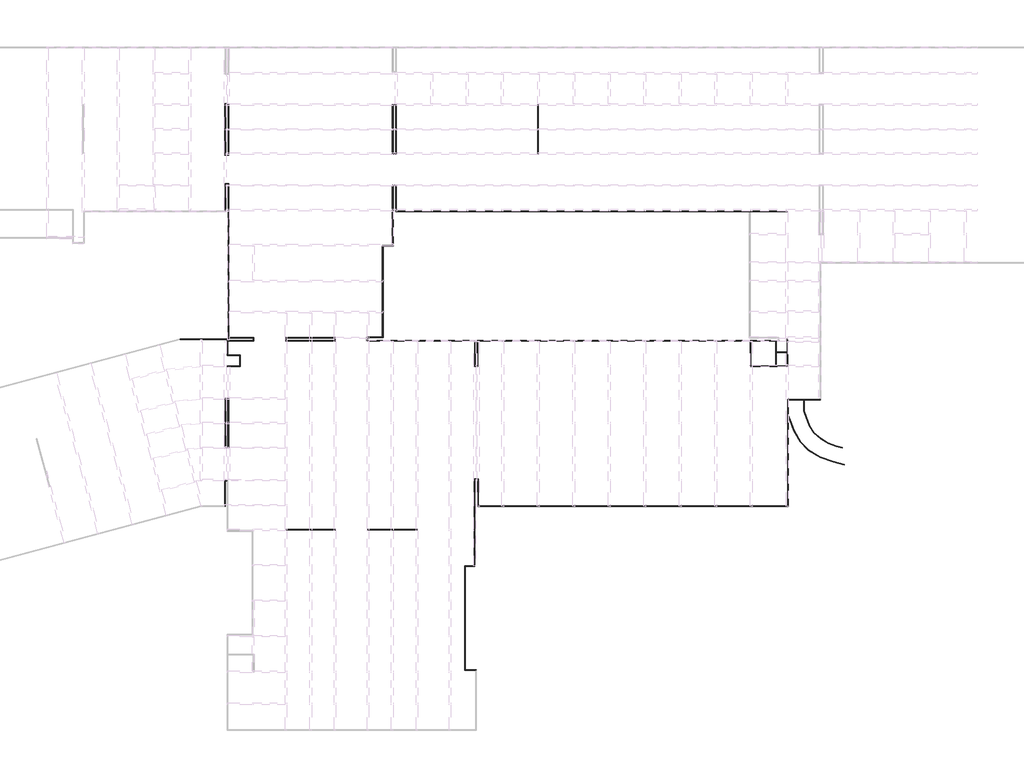
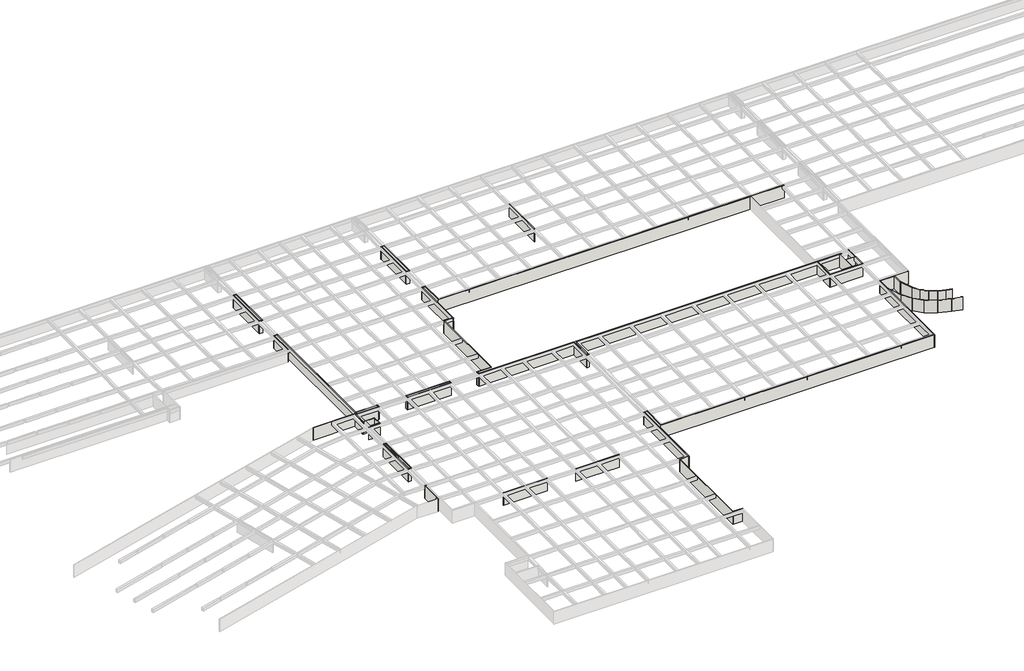
# One storey, part 2 of 14: 73 walls.
"""IFC4 building model written with IfcOpenShell, lengths in millimetres."""

import ifcopenshell
import ifcopenshell.guid

model = None  # the IFC model being written
_history = None  # IfcOwnerHistory: only IFC2X3 demands one
_inside = {}  # id of a spatial element -> (the spatial element, [elements in it])
_under = {}  # id of a project, library or spatial element -> (it, [spatial elements below it])
_declared = {}  # id of a project -> (the project, [libraries it declares])
_typed = {}  # id of a type object -> (the type object, [elements of that type])
_made_of = {}  # id of a material, layer set ... -> (it, [elements and type objects made of it])


def new_model(schema):
    """Start an empty IFC model of exactly this schema.

    Asked for "IFC4X3", IfcOpenShell would pick the latest addendum, in which some entities
    have other attributes; the version numbers below select the first issue.
    IFC2X3 requires an IfcOwnerHistory on every rooted entity: one is made here for all.
    """
    global model, _history
    if schema == "IFC4X3":
        model = ifcopenshell.file(schema_version=(4, 3, 0, 0))
    else:
        model = ifcopenshell.file(schema=schema)
    _inside.clear()
    _under.clear()
    _declared.clear()
    _typed.clear()
    _made_of.clear()
    _history = None
    if model.schema == "IFC2X3":
        org = make("IfcOrganization", Name="unknown")
        user = make(
            "IfcPersonAndOrganization",
            ThePerson=make("IfcPerson", FamilyName="unknown"),
            TheOrganization=org,
        )
        app = make(
            "IfcApplication",
            ApplicationDeveloper=org,
            Version="unknown",
            ApplicationFullName="unknown",
            ApplicationIdentifier="unknown",
        )
        _history = make(
            "IfcOwnerHistory",
            OwningUser=user,
            OwningApplication=app,
            ChangeAction="ADDED",
            CreationDate=0,
        )
    return model


def make(cls, **values):
    """One entity of the class cls with the attributes given. An attribute that is None is left unset."""
    return model.create_entity(
        cls, **{name: value for name, value in values.items() if value is not None}
    )


def rooted(cls, **values):
    """An entity with a GlobalId (a new one), such as an element, a storey or a relation."""
    return make(cls, GlobalId=ifcopenshell.guid.new(), OwnerHistory=_history, **values)


def si_unit(unit_type, name, prefix=None):
    """IfcSIUnit, for example si_unit("LENGTHUNIT", "METRE", prefix="MILLI")."""
    return make("IfcSIUnit", UnitType=unit_type, Prefix=prefix, Name=name)


def assignment(units):
    """IfcUnitAssignment: the units of a project."""
    return None if units is None else make("IfcUnitAssignment", Units=units)


def point(xyz):
    """IfcCartesianPoint."""
    return None if xyz is None else make("IfcCartesianPoint", Coordinates=xyz)


def direction(xyz):
    """IfcDirection."""
    return None if xyz is None else make("IfcDirection", DirectionRatios=xyz)


def frame(location, z_axis=None, x_axis=None):
    """IfcAxis2Placement3D, a coordinate frame: its origin and axes. An axis left out is left unset."""
    return make(
        "IfcAxis2Placement3D",
        Location=point(location),
        Axis=direction(z_axis),
        RefDirection=direction(x_axis),
    )


def origin():
    """The frame at (0, 0, 0) with its axes left unset."""
    return frame((0.0, 0.0, 0.0))


def origin_with_axes():
    """The frame at (0, 0, 0) with the z axis (0, 0, 1) and the x axis (1, 0, 0) written out."""
    return frame((0.0, 0.0, 0.0), z_axis=(0.0, 0.0, 1.0), x_axis=(1.0, 0.0, 0.0))


def place(relative_to, where):
    """IfcLocalPlacement: puts the frame where relative to a parent placement (None: the world)."""
    return make(
        "IfcLocalPlacement", PlacementRelTo=relative_to, RelativePlacement=where
    )


def context(
    kind, dimensions, precision=None, world=None, true_north=None, identifier=None
):
    """IfcGeometricRepresentationContext, for example the 3D "Model" context."""
    return make(
        "IfcGeometricRepresentationContext",
        ContextIdentifier=identifier,
        ContextType=kind,
        CoordinateSpaceDimension=dimensions,
        Precision=precision,
        WorldCoordinateSystem=world,
        TrueNorth=true_north,
    )


def project(units=None, contexts=None):
    """IfcProject with its units and contexts."""
    return rooted(
        "IfcProject",
        Name="project",
        RepresentationContexts=contexts,
        UnitsInContext=assignment(units),
    )


def spatial(cls, under=None, at=None, **own):
    """A site, building, storey or space (cls), placed at a placement, below another one or the project."""
    s = rooted(cls, ObjectPlacement=at, **own)
    if under is not None:
        _under.setdefault(under.id(), (under, []))[1].append(s)
    return s


def polyline(points):
    """IfcPolyline through the points."""
    return make("IfcPolyline", Points=[point(p) for p in points])


def outline(outer, holes=None, kind="AREA"):
    """IfcArbitraryClosedProfileDef: a profile drawn as a closed curve; with holes, ...WithVoids."""
    if holes is None:
        return make("IfcArbitraryClosedProfileDef", ProfileType=kind, OuterCurve=outer)
    return make(
        "IfcArbitraryProfileDefWithVoids",
        ProfileType=kind,
        OuterCurve=outer,
        InnerCurves=holes,
    )


def extrude(swept, where, along, depth):
    """IfcExtrudedAreaSolid: the profile swept, set in the frame where, extruded along a direction by depth."""
    return make(
        "IfcExtrudedAreaSolid",
        SweptArea=swept,
        Position=where,
        ExtrudedDirection=direction(along),
        Depth=depth,
    )


def faces_of(points, faces, orient=None, outer=None):
    """IfcFace entities. A face is a list of loops; a loop is a list of indices into points, from 0.

    orient and outer hold one flag for each loop. By default every Orientation is true, the
    first loop of a face is its IfcFaceOuterBound and the others are IfcFaceBound.
    """
    made = []
    for i, loops in enumerate(faces):
        bounds = []
        for j, loop in enumerate(loops):
            is_outer = j == 0 if outer is None else outer[i][j]
            bounds.append(
                make(
                    "IfcFaceOuterBound" if is_outer else "IfcFaceBound",
                    Bound=make("IfcPolyLoop", Polygon=[points[k] for k in loop]),
                    Orientation=True if orient is None else orient[i][j],
                )
            )
        made.append(make("IfcFace", Bounds=bounds))
    return made


def faceted_brep(points, faces, orient=None, outer=None, voids=None):
    """IfcFacetedBrep: a solid bounded by flat faces; with voids (closed shells), ...WithVoids."""
    shared = [point(p) for p in points]
    hull = make("IfcClosedShell", CfsFaces=faces_of(shared, faces, orient, outer))
    if voids is None:
        return make("IfcFacetedBrep", Outer=hull)
    return make(
        "IfcFacetedBrepWithVoids",
        Outer=hull,
        Voids=[
            make(cls, CfsFaces=faces_of(shared, fs, o, b)) for cls, fs, o, b in voids
        ],
    )


def shape(context_of_items, identifier, shape_type, items):
    """IfcShapeRepresentation: the items that make up one representation, for example the "Body"."""
    return make(
        "IfcShapeRepresentation",
        ContextOfItems=context_of_items,
        RepresentationIdentifier=identifier,
        RepresentationType=shape_type,
        Items=items,
    )


def made_of(thing, what):
    """Note that an element or type object is made of a material, layer set ...; save() writes the relation."""
    if what is not None:
        _made_of.setdefault(what.id(), (what, []))[1].append(thing)
    return thing


def element(
    cls,
    number,
    at=None,
    inside=None,
    cuts=None,
    type_object=None,
    material=None,
    context=None,
    identifier="Body",
    shape_type=None,
    held_by="IfcProductDefinitionShape",
    body=None,
    shapes=None,
    **own,
):
    """One element of the class cls, such as IfcWall. Its Tag is "e" and its number.

    at: its placement. inside: the storey or other place that contains it. cuts: it is an
    opening in that element (IfcRelVoidsElement). A single representation is given by context,
    identifier, shape_type and body (its items); several are given by shapes. held_by: the class
    of the entity that holds the representations. save() writes the other relations.
    """
    e = rooted(cls, Tag="e%d" % number, ObjectPlacement=at, **own)
    if body is not None:
        shapes = [shape(context, identifier, shape_type, body)]
    if shapes is not None:
        e.Representation = make(held_by, Representations=shapes)
    if inside is not None:
        _inside.setdefault(inside.id(), (inside, []))[1].append(e)
    if cuts is not None:
        rooted(
            "IfcRelVoidsElement", RelatingBuildingElement=cuts, RelatedOpeningElement=e
        )
    if type_object is not None:
        _typed.setdefault(type_object.id(), (type_object, []))[1].append(e)
    return made_of(e, material)


def aggregate(whole, parts):
    """IfcRelAggregates: a whole, such as a stair, and the parts it consists of."""
    return rooted("IfcRelAggregates", RelatingObject=whole, RelatedObjects=parts)


def save(model, path):
    """Write the relations noted so far, then the file.

    IfcRelAggregates (storeys below a building ...), IfcRelContainedInSpatialStructure (elements
    in a storey), IfcRelDefinesByType, IfcRelAssociatesMaterial and IfcRelDeclares: one each for
    every whole, place, type object, material and project.
    """
    for whole, parts in _under.values():
        aggregate(whole, parts)
    for where, things in _inside.values():
        rooted(
            "IfcRelContainedInSpatialStructure",
            RelatedElements=things,
            RelatingStructure=where,
        )
    for kind, things in _typed.values():
        rooted("IfcRelDefinesByType", RelatedObjects=things, RelatingType=kind)
    for what, things in _made_of.values():
        rooted("IfcRelAssociatesMaterial", RelatedObjects=things, RelatingMaterial=what)
    for by, libraries in _declared.values():
        rooted("IfcRelDeclares", RelatingContext=by, RelatedDefinitions=libraries)
    model.write(path)


model = new_model("IFC4")

# Units and contexts
model_context = context("Model", 3, world=origin())
ifc_project = project(units=[si_unit("LENGTHUNIT", "METRE", prefix="MILLI")], contexts=[model_context])

# Site, building, storey
site = spatial("IfcSite", under=ifc_project)
building = spatial("IfcBuilding", under=site)
storey = spatial("IfcBuildingStorey", under=building, Name="户型图", Elevation=0.0)

# Walls
placement = place(None, origin())
element("IfcWall", 1, ObjectType="所有墙体", at=placement, inside=storey, context=model_context, shape_type="Brep", body=[
    faceted_brep([(143467.2949044, -194796.0449275, 0.0), (136367.2949044, -194796.0449275, 0.0), (136367.2949044, -194796.0449275, 3300.0), (143467.2949044, -194796.0449275, 3300.0), (143467.2949044, -194916.0449275, 0.0), (143467.2949044, -194916.0449275, 3300.0), (140037.2949044, -194916.0449275, 3300.0), (139917.2949044, -194916.0449275, 3300.0), (136487.2949044, -194916.0449275, 3300.0), (136367.2949044, -194916.0449275, 3300.0), (136367.2949044, -194916.0449275, 0.0), (136487.2949044, -194916.0449275, 0.0), (139917.2949044, -194916.0449275, 0.0), (140037.2949044, -194916.0449275, 0.0)], [[[0, 1, 2, 3]], [[4, 5, 6, 7, 8, 9, 10, 11, 12, 13]], [[1, 0, 4, 13, 12, 11, 10]], [[3, 2, 9, 8, 7, 6, 5]], [[0, 3, 5, 4]], [[2, 1, 10, 9]]]),
])
element("IfcWall", 2, ObjectType="所有墙体", at=placement, inside=storey, context=model_context, shape_type="Brep", body=[
    faceted_brep([(136367.2949044, -194916.0449275, 0.0), (136367.2949044, -218198.950757, 0.0), (136367.2949044, -218318.950757, 0.0), (136367.2949044, -218318.950757, 3300.0), (136367.2949044, -218198.950757, 3300.0), (136367.2949044, -194916.0449275, 3300.0), (136487.2949044, -194916.0449275, 0.0), (136487.2949044, -194916.0449275, 3300.0), (136487.2949044, -198144.3728891, 3300.0), (136487.2949044, -198495.2294172, 3300.0), (136487.2949044, -218318.950757, 3300.0), (136487.2949044, -218318.950757, 0.0), (136487.2949044, -198495.2294172, 0.0), (136487.2949044, -198144.3728891, 0.0)], [[[0, 1, 2, 3, 4, 5]], [[6, 7, 8, 9, 10, 11, 12, 13]], [[2, 1, 0, 6, 13, 12, 11]], [[5, 4, 3, 10, 9, 8, 7]], [[0, 5, 7, 6]], [[3, 2, 11, 10]]]),
])
element("IfcWall", 3, ObjectType="所有墙体", at=placement, inside=storey, context=model_context, shape_type="Brep", body=[
    faceted_brep([(136367.2949044, -218198.950757, 0.0), (68337.2949044, -218198.950757, 0.0), (68217.2949044, -218198.950757, 0.0), (68217.2949044, -218198.950757, 3300.0), (68337.2949044, -218198.950757, 3300.0), (136367.2949044, -218198.950757, 3300.0), (136367.2949044, -218318.950757, 0.0), (136367.2949044, -218318.950757, 3300.0), (68217.2949044, -218318.950757, 3300.0), (68217.2949044, -218318.950757, 0.0)], [[[0, 1, 2, 3, 4, 5]], [[6, 7, 8, 9]], [[2, 1, 0, 6, 9]], [[5, 4, 3, 8, 7]], [[0, 5, 7, 6]], [[3, 2, 9, 8]]]),
])
element("IfcWall", 4, ObjectType="所有墙体", at=placement, inside=storey, context=model_context, shape_type="Brep", body=[
    faceted_brep([(68337.2949044, -218198.950757, 0.0), (68337.2949044, -212198.950757, 0.0), (68337.2949044, -212198.950757, 3300.0), (68337.2949044, -218198.950757, 3300.0), (68217.2949044, -218198.950757, 0.0), (68217.2949044, -218198.950757, 3300.0), (68217.2949044, -212318.950757, 3300.0), (68217.2949044, -212198.950757, 3300.0), (68217.2949044, -212198.950757, 0.0), (68217.2949044, -212318.950757, 0.0)], [[[0, 1, 2, 3]], [[4, 5, 6, 7, 8, 9]], [[1, 0, 4, 9, 8]], [[3, 2, 7, 6, 5]], [[0, 3, 5, 4]], [[2, 1, 8, 7]]]),
])
element("IfcWall", 5, ObjectType="所有墙体", at=placement, inside=storey, context=model_context, shape_type="Brep", body=[
    faceted_brep([(68217.2949044, -212198.950757, 0.0), (67517.2949044, -212198.950757, 0.0), (67517.2949044, -212198.950757, 3300.0), (68217.2949044, -212198.950757, 3300.0), (68217.2949044, -212318.950757, 0.0), (68217.2949044, -212318.950757, 3300.0), (67637.2949044, -212318.950757, 3300.0), (67517.2949044, -212318.950757, 3300.0), (67517.2949044, -212318.950757, 0.0), (67637.2949044, -212318.950757, 0.0)], [[[0, 1, 2, 3]], [[4, 5, 6, 7, 8, 9]], [[1, 0, 4, 9, 8]], [[3, 2, 7, 6, 5]], [[0, 3, 5, 4]], [[2, 1, 8, 7]]]),
])
element("IfcWall", 6, ObjectType="所有墙体", at=placement, inside=storey, context=model_context, shape_type="Brep", body=[
    faceted_brep([(67517.2949044, -212318.950757, 0.0), (67517.2949044, -231399.1116625, 0.0), (67517.2949044, -231519.1116625, 0.0), (67517.2949044, -231519.1116625, 3300.0), (67517.2949044, -231399.1116625, 3300.0), (67517.2949044, -212318.950757, 3300.0), (67637.2949044, -212318.950757, 0.0), (67637.2949044, -212318.950757, 3300.0), (67637.2949044, -231519.1116625, 3300.0), (67637.2949044, -231519.1116625, 0.0)], [[[0, 1, 2, 3, 4, 5]], [[6, 7, 8, 9]], [[2, 1, 0, 6, 9]], [[5, 4, 3, 8, 7]], [[0, 5, 7, 6]], [[3, 2, 9, 8]]]),
])
element("IfcWall", 7, ObjectType="所有墙体", at=placement, inside=storey, context=model_context, shape_type="Brep", body=[
    faceted_brep([(67517.2949044, -231399.1116625, 0.0), (65367.2949044, -231399.1116625, 0.0), (65367.2949044, -231399.1116625, 3300.0), (67517.2949044, -231399.1116625, 3300.0), (67517.2949044, -231519.1116625, 0.0), (67517.2949044, -231519.1116625, 3300.0), (65487.2949044, -231519.1116625, 3300.0), (65367.2949044, -231519.1116625, 3300.0), (65367.2949044, -231519.1116625, 0.0), (65487.2949044, -231519.1116625, 0.0)], [[[0, 1, 2, 3]], [[4, 5, 6, 7, 8, 9]], [[1, 0, 4, 9, 8]], [[3, 2, 7, 6, 5]], [[0, 3, 5, 4]], [[2, 1, 8, 7]]]),
])
element("IfcWall", 8, ObjectType="所有墙体", at=placement, inside=storey, context=model_context, shape_type="Brep", body=[
    faceted_brep([(65367.2949044, -231519.1116625, 0.0), (65367.2949044, -254333.1116625, 0.0), (65367.2949044, -254333.1116625, 3300.0), (65367.2949044, -231519.1116625, 3300.0), (65487.2949044, -231519.1116625, 0.0), (65487.2949044, -231519.1116625, 3300.0), (65487.2949044, -254213.1116625, 3300.0), (65487.2949044, -254333.1116625, 3300.0), (65487.2949044, -254333.1116625, 0.0), (65487.2949044, -254213.1116625, 0.0)], [[[0, 1, 2, 3]], [[4, 5, 6, 7, 8, 9]], [[1, 0, 4, 9, 8]], [[3, 2, 7, 6, 5]], [[0, 3, 5, 4]], [[2, 1, 8, 7]]]),
])
element("IfcWall", 9, ObjectType="所有墙体", at=placement, inside=storey, context=model_context, shape_type="Brep", body=[
    faceted_brep([(65487.2949044, -254333.1116625, 0.0), (67772.2743803, -254333.1116625, 0.0), (67892.2743803, -254333.1116625, 0.0), (67892.2743803, -254333.1116625, 3300.0), (67772.2743803, -254333.1116625, 3300.0), (65487.2949044, -254333.1116625, 3300.0), (65487.2949044, -254213.1116625, 0.0), (65487.2949044, -254213.1116625, 3300.0), (67892.2743803, -254213.1116625, 3300.0), (67892.2743803, -254213.1116625, 0.0)], [[[0, 1, 2, 3, 4, 5]], [[6, 7, 8, 9]], [[2, 1, 0, 6, 9]], [[5, 4, 3, 8, 7]], [[0, 5, 7, 6]], [[3, 2, 9, 8]]]),
])
element("IfcWall", 10, ObjectType="所有墙体", at=placement, inside=storey, context=model_context, shape_type="Brep", body=[
    faceted_brep([(13172.2743803, -212513.1116625, 0.0), (12672.2743803, -212513.1116625, 0.0), (12672.2743803, -212513.1116625, 3300.0), (13172.2743803, -212513.1116625, 3300.0), (13172.2743803, -212633.1116625, 0.0), (13172.2743803, -212633.1116625, 3300.0), (12792.2743803, -212633.1116625, 3300.0), (12672.2743803, -212633.1116625, 3300.0), (12672.2743803, -212633.1116625, 0.0), (12792.2743803, -212633.1116625, 0.0)], [[[0, 1, 2, 3]], [[4, 5, 6, 7, 8, 9]], [[1, 0, 4, 9, 8]], [[3, 2, 7, 6, 5]], [[0, 3, 5, 4]], [[2, 1, 8, 7]]]),
])
element("IfcWall", 11, ObjectType="所有墙体", at=placement, inside=storey, context=model_context, shape_type="Brep", body=[
    faceted_brep([(12672.2743803, -212633.1116625, 0.0), (12672.2743803, -218205.2956278, 0.0), (12672.2743803, -218325.2956278, 0.0), (12672.2743803, -218325.2956278, 3300.0), (12672.2743803, -218205.2956278, 3300.0), (12672.2743803, -212633.1116625, 3300.0), (12792.2743803, -212633.1116625, 0.0), (12792.2743803, -212633.1116625, 3300.0), (12792.2743803, -218325.2956278, 3300.0), (12792.2743803, -218325.2956278, 0.0)], [[[0, 1, 2, 3, 4, 5]], [[6, 7, 8, 9]], [[2, 1, 0, 6, 9]], [[5, 4, 3, 8, 7]], [[0, 5, 7, 6]], [[3, 2, 9, 8]]]),
])
element("IfcWall", 12, ObjectType="所有墙体", at=placement, inside=storey, context=model_context, shape_type="Brep", body=[
    faceted_brep([(2737.534582, -181627.3751505, 0.0), (13167.2949044, -181627.3751505, 0.0), (13287.2949044, -181627.3751505, 0.0), (13589.6354322, -181627.3751505, 0.0), (13589.6354322, -181627.3751505, 3300.0), (13287.2949044, -181627.3751505, 3300.0), (13167.2949044, -181627.3751505, 3300.0), (2737.534582, -181627.3751505, 3300.0), (2721.7362823, -181507.3751505, 0.0), (2721.7362823, -181507.3751505, 3300.0), (13469.6354322, -181507.3751505, 3300.0), (13589.6354322, -181507.3751505, 3300.0), (13589.6354322, -181507.3751505, 0.0), (13469.6354322, -181507.3751505, 0.0)], [[[0, 1, 2, 3, 4, 5, 6, 7]], [[8, 9, 10, 11, 12, 13]], [[3, 2, 1, 0, 8, 13, 12]], [[7, 6, 5, 4, 11, 10, 9]], [[0, 7, 9, 8]], [[4, 3, 12, 11]]]),
])
element("IfcWall", 13, ObjectType="所有墙体", at=placement, inside=storey, context=model_context, shape_type="Brep", body=[
    faceted_brep([(13589.6354322, -181507.3751505, 0.0), (13589.6354322, -181254.9655707, 0.0), (13589.6354322, -181134.9655707, 0.0), (13589.6354322, -147307.3751505, 0.0), (13589.6354322, -147307.3751505, 3300.0), (13589.6354322, -181134.9655707, 3300.0), (13589.6354322, -181254.9655707, 3300.0), (13589.6354322, -181507.3751505, 3300.0), (13469.6354322, -181507.3751505, 0.0), (13469.6354322, -181507.3751505, 3300.0), (13469.6354322, -147427.3751505, 3300.0), (13469.6354322, -147307.3751505, 3300.0), (13469.6354322, -147307.3751505, 0.0), (13469.6354322, -147427.3751505, 0.0)], [[[0, 1, 2, 3, 4, 5, 6, 7]], [[8, 9, 10, 11, 12, 13]], [[3, 2, 1, 0, 8, 13, 12]], [[7, 6, 5, 4, 11, 10, 9]], [[0, 7, 9, 8]], [[4, 3, 12, 11]]]),
])
element("IfcWall", 14, ObjectType="所有墙体", at=placement, inside=storey, context=model_context, shape_type="Brep", body=[
    faceted_brep([(13469.6354322, -147307.3751505, 0.0), (12717.2949044, -147307.3751505, 0.0), (12717.2949044, -147307.3751505, 3300.0), (13469.6354322, -147307.3751505, 3300.0), (13469.6354322, -147427.3751505, 0.0), (13469.6354322, -147427.3751505, 3300.0), (12837.2949044, -147427.3751505, 3300.0), (12717.2949044, -147427.3751505, 3300.0), (12717.2949044, -147427.3751505, 0.0), (12837.2949044, -147427.3751505, 0.0)], [[[0, 1, 2, 3]], [[4, 5, 6, 7, 8, 9]], [[1, 0, 4, 9, 8]], [[3, 2, 7, 6, 5]], [[0, 3, 5, 4]], [[2, 1, 8, 7]]]),
])
element("IfcWall", 15, ObjectType="所有墙体", at=placement, inside=storey, context=model_context, shape_type="Brep", body=[
    faceted_brep([(12717.2949044, -147427.3751505, 0.0), (12717.2949044, -153307.3751505, 0.0), (12717.2949044, -153427.3751505, 0.0), (12717.2949044, -153427.3751505, 3300.0), (12717.2949044, -153307.3751505, 3300.0), (12717.2949044, -147427.3751505, 3300.0), (12837.2949044, -147427.3751505, 0.0), (12837.2949044, -147427.3751505, 3300.0), (12837.2949044, -153427.3751505, 3300.0), (12837.2949044, -153427.3751505, 0.0)], [[[0, 1, 2, 3, 4, 5]], [[6, 7, 8, 9]], [[2, 1, 0, 6, 9]], [[5, 4, 3, 8, 7]], [[0, 5, 7, 6]], [[3, 2, 9, 8]]]),
])
element("IfcWall", 16, ObjectType="所有墙体", at=placement, inside=storey, context=model_context, shape_type="Brep", body=[
    faceted_brep([(12767.2949044, -194498.950757, 0.0), (12767.2949044, -205418.950757, 0.0), (12767.2949044, -205418.950757, 3300.0), (12767.2949044, -194498.950757, 3300.0), (12887.2949044, -194498.950757, 0.0), (12887.2949044, -194498.950757, 3300.0), (12887.2949044, -194618.950757, 3300.0), (12887.2949044, -205298.950757, 3300.0), (12887.2949044, -205418.950757, 3300.0), (12887.2949044, -205418.950757, 0.0), (12887.2949044, -205298.950757, 0.0), (12887.2949044, -194618.950757, 0.0)], [[[0, 1, 2, 3]], [[4, 5, 6, 7, 8, 9, 10, 11]], [[1, 0, 4, 11, 10, 9]], [[3, 2, 8, 7, 6, 5]], [[2, 1, 9, 8]], [[0, 3, 5, 4]]]),
])
element("IfcWall", 17, ObjectType="所有墙体", at=placement, inside=storey, context=model_context, shape_type="Brep", body=[
    faceted_brep([(12887.2949044, -205418.950757, 0.0), (13487.2949044, -205418.950757, 0.0), (13487.2949044, -205418.950757, 3300.0), (12887.2949044, -205418.950757, 3300.0), (12887.2949044, -205298.950757, 0.0), (12887.2949044, -205298.950757, 3300.0), (13367.2949044, -205298.950757, 3300.0), (13487.2949044, -205298.950757, 3300.0), (13487.2949044, -205298.950757, 0.0), (13367.2949044, -205298.950757, 0.0)], [[[0, 1, 2, 3]], [[4, 5, 6, 7, 8, 9]], [[1, 0, 4, 9, 8]], [[3, 2, 7, 6, 5]], [[0, 3, 5, 4]], [[2, 1, 8, 7]]]),
])
element("IfcWall", 18, ObjectType="所有墙体", at=placement, inside=storey, context=model_context, shape_type="Brep", body=[
    faceted_brep([(13487.2949044, -205298.950757, 0.0), (13487.2949044, -194498.950757, 0.0), (13487.2949044, -194498.950757, 3300.0), (13487.2949044, -205298.950757, 3300.0), (13367.2949044, -205298.950757, 0.0), (13367.2949044, -205298.950757, 3300.0), (13367.2949044, -194618.950757, 3300.0), (13367.2949044, -194498.950757, 3300.0), (13367.2949044, -194498.950757, 0.0), (13367.2949044, -194618.950757, 0.0)], [[[0, 1, 2, 3]], [[4, 5, 6, 7, 8, 9]], [[1, 0, 4, 9, 8]], [[3, 2, 7, 6, 5]], [[0, 3, 5, 4]], [[2, 1, 8, 7]]]),
])
element("IfcWall", 19, ObjectType="所有墙体", at=placement, inside=storey, context=model_context, shape_type="SweptSolid", body=[
    extrude(outline(polyline([(12887.2949044, -194498.950757), (13367.2949044, -194498.950757), (13367.2949044, -194618.950757), (12887.2949044, -194618.950757), (12887.2949044, -194498.950757)])), origin_with_axes(), (0.0, 0.0, 1.0), 3300.0),
])
element("IfcWall", 20, ObjectType="所有墙体", at=placement, inside=storey, context=model_context, shape_type="Brep", body=[
    faceted_brep([(13227.2949044, -187518.950757, 0.0), (16086.994268, -187518.950757, 0.0), (16086.994268, -187518.950757, 3300.0), (13227.2949044, -187518.950757, 3300.0), (13227.2949044, -187398.950757, 0.0), (13227.2949044, -187398.950757, 3300.0), (15966.994268, -187398.950757, 3300.0), (16086.994268, -187398.950757, 3300.0), (16086.994268, -187398.950757, 0.0), (15966.994268, -187398.950757, 0.0)], [[[0, 1, 2, 3]], [[4, 5, 6, 7, 8, 9]], [[1, 0, 4, 9, 8]], [[3, 2, 7, 6, 5]], [[0, 3, 5, 4]], [[2, 1, 8, 7]]]),
])
element("IfcWall", 21, ObjectType="所有墙体", at=placement, inside=storey, context=model_context, shape_type="Brep", body=[
    faceted_brep([(16086.994268, -187398.950757, 0.0), (16086.994268, -184998.950757, 0.0), (16086.994268, -184998.950757, 3300.0), (16086.994268, -187398.950757, 3300.0), (15966.994268, -187398.950757, 0.0), (15966.994268, -187398.950757, 3300.0), (15966.994268, -185118.950757, 3300.0), (15966.994268, -184998.950757, 3300.0), (15966.994268, -184998.950757, 0.0), (15966.994268, -185118.950757, 0.0)], [[[0, 1, 2, 3]], [[4, 5, 6, 7, 8, 9]], [[1, 0, 4, 9, 8]], [[3, 2, 7, 6, 5]], [[0, 3, 5, 4]], [[2, 1, 8, 7]]]),
])
element("IfcWall", 22, ObjectType="所有墙体", at=placement, inside=storey, context=model_context, shape_type="Brep", body=[
    faceted_brep([(15966.994268, -184998.950757, 0.0), (13287.2949044, -184998.950757, 0.0), (13167.2949044, -184998.950757, 0.0), (13167.2949044, -184998.950757, 3300.0), (13287.2949044, -184998.950757, 3300.0), (15966.994268, -184998.950757, 3300.0), (15966.994268, -185118.950757, 0.0), (15966.994268, -185118.950757, 3300.0), (13167.2949044, -185118.950757, 3300.0), (13167.2949044, -185118.950757, 0.0)], [[[0, 1, 2, 3, 4, 5]], [[6, 7, 8, 9]], [[2, 1, 0, 6, 9]], [[5, 4, 3, 8, 7]], [[0, 5, 7, 6]], [[3, 2, 9, 8]]]),
])
element("IfcWall", 23, ObjectType="所有墙体", at=placement, inside=storey, context=model_context, shape_type="Brep", body=[
    faceted_brep([(13287.2949044, -184998.950757, 0.0), (13287.2949044, -181918.950757, 0.0), (13287.2949044, -181798.950757, 0.0), (13287.2949044, -181627.3751505, 0.0), (13287.2949044, -181627.3751505, 3300.0), (13287.2949044, -181798.950757, 3300.0), (13287.2949044, -181918.950757, 3300.0), (13287.2949044, -184998.950757, 3300.0), (13167.2949044, -184998.950757, 0.0), (13167.2949044, -184998.950757, 3300.0), (13167.2949044, -181627.3751505, 3300.0), (13167.2949044, -181627.3751505, 0.0)], [[[0, 1, 2, 3, 4, 5, 6, 7]], [[8, 9, 10, 11]], [[3, 2, 1, 0, 8, 11]], [[7, 6, 5, 4, 10, 9]], [[0, 7, 9, 8]], [[4, 3, 11, 10]]]),
])
element("IfcWall", 24, ObjectType="所有墙体", at=placement, inside=storey, context=model_context, shape_type="Brep", body=[
    faceted_brep([(13589.6354322, -181254.9655707, 0.0), (18882.7925222, -181254.9655707, 0.0), (19002.7925222, -181254.9655707, 0.0), (19002.7925222, -181254.9655707, 3300.0), (18882.7925222, -181254.9655707, 3300.0), (13589.6354322, -181254.9655707, 3300.0), (13589.6354322, -181134.9655707, 0.0), (13589.6354322, -181134.9655707, 3300.0), (19002.7925222, -181134.9655707, 3300.0), (19002.7925222, -181134.9655707, 0.0)], [[[0, 1, 2, 3, 4, 5]], [[6, 7, 8, 9]], [[2, 1, 0, 6, 9]], [[5, 4, 3, 8, 7]], [[0, 5, 7, 6]], [[3, 2, 9, 8]]]),
])
element("IfcWall", 25, ObjectType="所有墙体", at=placement, inside=storey, context=model_context, shape_type="Brep", body=[
    faceted_brep([(18882.7925222, -181254.9655707, 0.0), (18882.7925222, -181798.950757, 0.0), (18882.7925222, -181918.950757, 0.0), (18882.7925222, -181918.950757, 3300.0), (18882.7925222, -181798.950757, 3300.0), (18882.7925222, -181254.9655707, 3300.0), (19002.7925222, -181254.9655707, 0.0), (19002.7925222, -181254.9655707, 3300.0), (19002.7925222, -181918.950757, 3300.0), (19002.7925222, -181918.950757, 0.0)], [[[0, 1, 2, 3, 4, 5]], [[6, 7, 8, 9]], [[2, 1, 0, 6, 9]], [[5, 4, 3, 8, 7]], [[0, 5, 7, 6]], [[3, 2, 9, 8]]]),
])
element("IfcWall", 26, ObjectType="所有墙体", at=placement, inside=storey, context=model_context, shape_type="SweptSolid", body=[
    extrude(outline(polyline([(13287.2949044, -181798.950757), (18882.7925222, -181798.950757), (18882.7925222, -181918.950757), (13287.2949044, -181918.950757), (13287.2949044, -181798.950757)])), origin_with_axes(), (0.0, 0.0, 1.0), 3300.0),
])
element("IfcWall", 27, ObjectType="所有墙体", at=placement, inside=storey, context=model_context, shape_type="Brep", body=[
    faceted_brep([(26067.2949044, -181184.9655707, 0.0), (26067.2949044, -181918.950757, 0.0), (26067.2949044, -181918.950757, 3300.0), (26067.2949044, -181184.9655707, 3300.0), (26187.2949044, -181184.9655707, 0.0), (26187.2949044, -181184.9655707, 3300.0), (26187.2949044, -181304.9655707, 3300.0), (26187.2949044, -181798.950757, 3300.0), (26187.2949044, -181918.950757, 3300.0), (26187.2949044, -181918.950757, 0.0), (26187.2949044, -181798.950757, 0.0), (26187.2949044, -181304.9655707, 0.0)], [[[0, 1, 2, 3]], [[4, 5, 6, 7, 8, 9, 10, 11]], [[1, 0, 4, 11, 10, 9]], [[3, 2, 8, 7, 6, 5]], [[2, 1, 9, 8]], [[0, 3, 5, 4]]]),
])
element("IfcWall", 28, ObjectType="所有墙体", at=placement, inside=storey, context=model_context, shape_type="Brep", body=[
    faceted_brep([(26187.2949044, -181918.950757, 0.0), (36992.3410651, -181918.950757, 0.0), (36992.3410651, -181918.950757, 3300.0), (26187.2949044, -181918.950757, 3300.0), (26187.2949044, -181798.950757, 0.0), (26187.2949044, -181798.950757, 3300.0), (36872.3410651, -181798.950757, 3300.0), (36992.3410651, -181798.950757, 3300.0), (36992.3410651, -181798.950757, 0.0), (36872.3410651, -181798.950757, 0.0)], [[[0, 1, 2, 3]], [[4, 5, 6, 7, 8, 9]], [[1, 0, 4, 9, 8]], [[3, 2, 7, 6, 5]], [[0, 3, 5, 4]], [[2, 1, 8, 7]]]),
])
element("IfcWall", 29, ObjectType="所有墙体", at=placement, inside=storey, context=model_context, shape_type="Brep", body=[
    faceted_brep([(36992.3410651, -181798.950757, 0.0), (36992.3410651, -181184.9655707, 0.0), (36992.3410651, -181184.9655707, 3300.0), (36992.3410651, -181798.950757, 3300.0), (36872.3410651, -181798.950757, 0.0), (36872.3410651, -181798.950757, 3300.0), (36872.3410651, -181304.9655707, 3300.0), (36872.3410651, -181184.9655707, 3300.0), (36872.3410651, -181184.9655707, 0.0), (36872.3410651, -181304.9655707, 0.0)], [[[0, 1, 2, 3]], [[4, 5, 6, 7, 8, 9]], [[1, 0, 4, 9, 8]], [[3, 2, 7, 6, 5]], [[0, 3, 5, 4]], [[2, 1, 8, 7]]]),
])
element("IfcWall", 30, ObjectType="所有墙体", at=placement, inside=storey, context=model_context, shape_type="SweptSolid", body=[
    extrude(outline(polyline([(26187.2949044, -181184.9655707), (36872.3410651, -181184.9655707), (36872.3410651, -181304.9655707), (26187.2949044, -181304.9655707), (26187.2949044, -181184.9655707)])), origin_with_axes(), (0.0, 0.0, 1.0), 3300.0),
])
element("IfcWall", 31, ObjectType="所有墙体", at=placement, inside=storey, context=model_context, shape_type="Brep", body=[
    faceted_brep([(47436.5330009, -181024.9655707, 0.0), (47316.5330009, -181024.9655707, 0.0), (43867.2949044, -181024.9655707, 0.0), (43867.2949044, -181024.9655707, 3300.0), (47316.5330009, -181024.9655707, 3300.0), (47436.5330009, -181024.9655707, 3300.0), (47436.5330009, -181144.9655707, 0.0), (47436.5330009, -181144.9655707, 3300.0), (43987.2949044, -181144.9655707, 3300.0), (43867.2949044, -181144.9655707, 3300.0), (43867.2949044, -181144.9655707, 0.0), (43987.2949044, -181144.9655707, 0.0)], [[[0, 1, 2, 3, 4, 5]], [[6, 7, 8, 9, 10, 11]], [[2, 1, 0, 6, 11, 10]], [[5, 4, 3, 9, 8, 7]], [[3, 2, 10, 9]], [[0, 5, 7, 6]]]),
])
element("IfcWall", 32, ObjectType="所有墙体", at=placement, inside=storey, context=model_context, shape_type="Brep", body=[
    faceted_brep([(43867.2949044, -181144.9655707, 0.0), (43867.2949044, -181968.950757, 0.0), (43867.2949044, -181968.950757, 3300.0), (43867.2949044, -181144.9655707, 3300.0), (43987.2949044, -181144.9655707, 0.0), (43987.2949044, -181144.9655707, 3300.0), (43987.2949044, -181848.950757, 3300.0), (43987.2949044, -181968.950757, 3300.0), (43987.2949044, -181968.950757, 0.0), (43987.2949044, -181848.950757, 0.0)], [[[0, 1, 2, 3]], [[4, 5, 6, 7, 8, 9]], [[1, 0, 4, 9, 8]], [[3, 2, 7, 6, 5]], [[0, 3, 5, 4]], [[2, 1, 8, 7]]]),
])
element("IfcWall", 33, ObjectType="所有墙体", at=placement, inside=storey, context=model_context, shape_type="Brep", body=[
    faceted_brep([(43987.2949044, -181968.950757, 0.0), (67567.2949044, -181968.950757, 0.0), (67687.2949044, -181968.950757, 0.0), (67687.2949044, -181968.950757, 3300.0), (67567.2949044, -181968.950757, 3300.0), (43987.2949044, -181968.950757, 3300.0), (43987.2949044, -181848.950757, 0.0), (43987.2949044, -181848.950757, 3300.0), (67687.2949044, -181848.950757, 3300.0), (67687.2949044, -181848.950757, 0.0)], [[[0, 1, 2, 3, 4, 5]], [[6, 7, 8, 9]], [[2, 1, 0, 6, 9]], [[5, 4, 3, 8, 7]], [[0, 5, 7, 6]], [[3, 2, 9, 8]]]),
])
element("IfcWall", 34, ObjectType="所有墙体", at=placement, inside=storey, context=model_context, shape_type="Brep", body=[
    faceted_brep([(67567.2949044, -181968.950757, 0.0), (67567.2949044, -187518.950757, 0.0), (67567.2949044, -187518.950757, 3300.0), (67567.2949044, -181968.950757, 3300.0), (67687.2949044, -181968.950757, 0.0), (67687.2949044, -181968.950757, 3300.0), (67687.2949044, -187398.950757, 3300.0), (67687.2949044, -187518.950757, 3300.0), (67687.2949044, -187518.950757, 0.0), (67687.2949044, -187398.950757, 0.0)], [[[0, 1, 2, 3]], [[4, 5, 6, 7, 8, 9]], [[1, 0, 4, 9, 8]], [[3, 2, 7, 6, 5]], [[0, 3, 5, 4]], [[2, 1, 8, 7]]]),
])
element("IfcWall", 35, ObjectType="所有墙体", at=placement, inside=storey, context=model_context, shape_type="Brep", body=[
    faceted_brep([(67687.2949044, -187518.950757, 0.0), (68228.3552546, -187518.950757, 0.0), (68228.3552546, -187518.950757, 3300.0), (67687.2949044, -187518.950757, 3300.0), (67687.2949044, -187398.950757, 0.0), (67687.2949044, -187398.950757, 3300.0), (68108.3552546, -187398.950757, 3300.0), (68228.3552546, -187398.950757, 3300.0), (68228.3552546, -187398.950757, 0.0), (68108.3552546, -187398.950757, 0.0)], [[[0, 1, 2, 3]], [[4, 5, 6, 7, 8, 9]], [[1, 0, 4, 9, 8]], [[3, 2, 7, 6, 5]], [[0, 3, 5, 4]], [[2, 1, 8, 7]]]),
])
element("IfcWall", 36, ObjectType="所有墙体", at=placement, inside=storey, context=model_context, shape_type="Brep", body=[
    faceted_brep([(68228.3552546, -187398.950757, 0.0), (68228.3552546, -181968.950757, 0.0), (68228.3552546, -181848.950757, 0.0), (68228.3552546, -181848.950757, 3300.0), (68228.3552546, -181968.950757, 3300.0), (68228.3552546, -187398.950757, 3300.0), (68108.3552546, -187398.950757, 0.0), (68108.3552546, -187398.950757, 3300.0), (68108.3552546, -181848.950757, 3300.0), (68108.3552546, -181848.950757, 0.0)], [[[0, 1, 2, 3, 4, 5]], [[6, 7, 8, 9]], [[2, 1, 0, 6, 9]], [[5, 4, 3, 8, 7]], [[0, 5, 7, 6]], [[3, 2, 9, 8]]]),
])
element("IfcWall", 37, ObjectType="所有墙体", at=placement, inside=storey, context=model_context, shape_type="Brep", body=[
    faceted_brep([(68228.3552546, -181968.950757, 0.0), (128167.631745, -181968.950757, 0.0), (128287.631745, -181968.950757, 0.0), (133768.0603935, -181968.950757, 0.0), (133888.0603935, -181968.950757, 0.0), (134428.3552546, -181968.950757, 0.0), (134428.3552546, -181968.950757, 3300.0), (133888.0603935, -181968.950757, 3300.0), (133768.0603935, -181968.950757, 3300.0), (128287.631745, -181968.950757, 3300.0), (128167.631745, -181968.950757, 3300.0), (68228.3552546, -181968.950757, 3300.0), (68228.3552546, -181848.950757, 0.0), (68228.3552546, -181848.950757, 3300.0), (134308.3552546, -181848.950757, 3300.0), (134428.3552546, -181848.950757, 3300.0), (134428.3552546, -181848.950757, 0.0), (134308.3552546, -181848.950757, 0.0)], [[[0, 1, 2, 3, 4, 5, 6, 7, 8, 9, 10, 11]], [[12, 13, 14, 15, 16, 17]], [[5, 4, 3, 2, 1, 0, 12, 17, 16]], [[11, 10, 9, 8, 7, 6, 15, 14, 13]], [[0, 11, 13, 12]], [[6, 5, 16, 15]]]),
])
element("IfcWall", 38, ObjectType="所有墙体", at=placement, inside=storey, context=model_context, shape_type="Brep", body=[
    faceted_brep([(50267.2949044, -153418.950757, 0.0), (127967.2949044, -153418.950757, 0.0), (128087.2949044, -153418.950757, 0.0), (136427.2949044, -153418.950757, 0.0), (136427.2949044, -153418.950757, 3300.0), (128087.2949044, -153418.950757, 3300.0), (127967.2949044, -153418.950757, 3300.0), (50267.2949044, -153418.950757, 3300.0), (50267.2949044, -153298.950757, 0.0), (50267.2949044, -153298.950757, 3300.0), (50387.2949044, -153298.950757, 3300.0), (136427.2949044, -153298.950757, 3300.0), (136427.2949044, -153298.950757, 0.0), (50387.2949044, -153298.950757, 0.0)], [[[0, 1, 2, 3, 4, 5, 6, 7]], [[8, 9, 10, 11, 12, 13]], [[3, 2, 1, 0, 8, 13, 12]], [[4, 3, 12, 11]], [[7, 6, 5, 4, 11, 10, 9]], [[0, 7, 9, 8]]]),
])
element("IfcWall", 39, ObjectType="所有墙体", at=placement, inside=storey, context=model_context, shape_type="Brep", body=[
    faceted_brep([(50387.2949044, -153298.950757, 0.0), (50387.2949044, -147598.950757, 0.0), (50387.2949044, -147598.950757, 3300.0), (50387.2949044, -153298.950757, 3300.0), (50267.2949044, -153298.950757, 0.0), (50267.2949044, -153298.950757, 3300.0), (50267.2949044, -147718.950757, 3300.0), (50267.2949044, -147598.950757, 3300.0), (50267.2949044, -147598.950757, 0.0), (50267.2949044, -147718.950757, 0.0)], [[[0, 1, 2, 3]], [[4, 5, 6, 7, 8, 9]], [[1, 0, 4, 9, 8]], [[3, 2, 7, 6, 5]], [[0, 3, 5, 4]], [[2, 1, 8, 7]]]),
])
element("IfcWall", 40, ObjectType="所有墙体", at=placement, inside=storey, context=model_context, shape_type="Brep", body=[
    faceted_brep([(50267.2949044, -147598.950757, 0.0), (49516.5330009, -147598.950757, 0.0), (49516.5330009, -147598.950757, 3300.0), (50267.2949044, -147598.950757, 3300.0), (50267.2949044, -147718.950757, 0.0), (50267.2949044, -147718.950757, 3300.0), (49636.5330009, -147718.950757, 3300.0), (49516.5330009, -147718.950757, 3300.0), (49516.5330009, -147718.950757, 0.0), (49636.5330009, -147718.950757, 0.0)], [[[0, 1, 2, 3]], [[4, 5, 6, 7, 8, 9]], [[1, 0, 4, 9, 8]], [[3, 2, 7, 6, 5]], [[0, 3, 5, 4]], [[2, 1, 8, 7]]]),
])
element("IfcWall", 41, ObjectType="所有墙体", at=placement, inside=storey, context=model_context, shape_type="Brep", body=[
    faceted_brep([(49516.5330009, -147718.950757, 0.0), (49516.5330009, -160898.950757, 0.0), (49516.5330009, -161018.950757, 0.0), (49516.5330009, -161018.950757, 3300.0), (49516.5330009, -160898.950757, 3300.0), (49516.5330009, -147718.950757, 3300.0), (49636.5330009, -147718.950757, 0.0), (49636.5330009, -147718.950757, 3300.0), (49636.5330009, -161018.950757, 3300.0), (49636.5330009, -161018.950757, 0.0)], [[[0, 1, 2, 3, 4, 5]], [[6, 7, 8, 9]], [[2, 1, 0, 6, 9]], [[5, 4, 3, 8, 7]], [[0, 5, 7, 6]], [[3, 2, 9, 8]]]),
])
element("IfcWall", 42, ObjectType="所有墙体", at=placement, inside=storey, context=model_context, shape_type="Brep", body=[
    faceted_brep([(49516.5330009, -160898.950757, 0.0), (47316.5330009, -160898.950757, 0.0), (47316.5330009, -160898.950757, 3300.0), (49516.5330009, -160898.950757, 3300.0), (49516.5330009, -161018.950757, 0.0), (49516.5330009, -161018.950757, 3300.0), (47436.5330009, -161018.950757, 3300.0), (47316.5330009, -161018.950757, 3300.0), (47316.5330009, -161018.950757, 0.0), (47436.5330009, -161018.950757, 0.0)], [[[0, 1, 2, 3]], [[4, 5, 6, 7, 8, 9]], [[1, 0, 4, 9, 8]], [[3, 2, 7, 6, 5]], [[0, 3, 5, 4]], [[2, 1, 8, 7]]]),
])
element("IfcWall", 43, ObjectType="所有墙体", at=placement, inside=storey, context=model_context, shape_type="SweptSolid", body=[
    extrude(outline(polyline([(47316.5330009, -181024.9655707), (47316.5330009, -161018.950757), (47436.5330009, -161018.950757), (47436.5330009, -181024.9655707), (47316.5330009, -181024.9655707)])), origin_with_axes(), (0.0, 0.0, 1.0), 3300.0),
])
element("IfcWall", 44, ObjectType="所有墙体", at=placement, inside=storey, context=model_context, shape_type="Brep", body=[
    faceted_brep([(12711.7961793, -141080.0179086, 0.0), (13537.2949044, -141080.0179086, 0.0), (13537.2949044, -141080.0179086, 3300.0), (12711.7961793, -141080.0179086, 3300.0), (12711.7961793, -140960.0179086, 0.0), (12711.7961793, -140960.0179086, 3300.0), (12831.7961793, -140960.0179086, 3300.0), (13417.2949044, -140960.0179086, 3300.0), (13537.2949044, -140960.0179086, 3300.0), (13537.2949044, -140960.0179086, 0.0), (13417.2949044, -140960.0179086, 0.0), (12831.7961793, -140960.0179086, 0.0)], [[[0, 1, 2, 3]], [[4, 5, 6, 7, 8, 9, 10, 11]], [[1, 0, 4, 11, 10, 9]], [[3, 2, 8, 7, 6, 5]], [[2, 1, 9, 8]], [[0, 3, 5, 4]]]),
])
element("IfcWall", 45, ObjectType="所有墙体", at=placement, inside=storey, context=model_context, shape_type="Brep", body=[
    faceted_brep([(13537.2949044, -140960.0179086, 0.0), (13537.2949044, -129760.0179086, 0.0), (13537.2949044, -129760.0179086, 3300.0), (13537.2949044, -140960.0179086, 3300.0), (13417.2949044, -140960.0179086, 0.0), (13417.2949044, -140960.0179086, 3300.0), (13417.2949044, -129880.0179086, 3300.0), (13417.2949044, -129760.0179086, 3300.0), (13417.2949044, -129760.0179086, 0.0), (13417.2949044, -129880.0179086, 0.0)], [[[0, 1, 2, 3]], [[4, 5, 6, 7, 8, 9]], [[1, 0, 4, 9, 8]], [[3, 2, 7, 6, 5]], [[0, 3, 5, 4]], [[2, 1, 8, 7]]]),
])
element("IfcWall", 46, ObjectType="所有墙体", at=placement, inside=storey, context=model_context, shape_type="Brep", body=[
    faceted_brep([(13417.2949044, -129760.0179086, 0.0), (12711.7961793, -129760.0179086, 0.0), (12711.7961793, -129760.0179086, 3300.0), (13417.2949044, -129760.0179086, 3300.0), (13417.2949044, -129880.0179086, 0.0), (13417.2949044, -129880.0179086, 3300.0), (12831.7961793, -129880.0179086, 3300.0), (12711.7961793, -129880.0179086, 3300.0), (12711.7961793, -129880.0179086, 0.0), (12831.7961793, -129880.0179086, 0.0)], [[[0, 1, 2, 3]], [[4, 5, 6, 7, 8, 9]], [[1, 0, 4, 9, 8]], [[3, 2, 7, 6, 5]], [[0, 3, 5, 4]], [[2, 1, 8, 7]]]),
])
element("IfcWall", 47, ObjectType="所有墙体", at=placement, inside=storey, context=model_context, shape_type="SweptSolid", body=[
    extrude(outline(polyline([(12711.7961793, -140960.0179086), (12711.7961793, -129880.0179086), (12831.7961793, -129880.0179086), (12831.7961793, -140960.0179086), (12711.7961793, -140960.0179086)])), origin_with_axes(), (0.0, 0.0, 1.0), 3300.0),
])
element("IfcWall", 48, ObjectType="所有墙体", at=placement, inside=storey, context=model_context, shape_type="Brep", body=[
    faceted_brep([(49516.5330009, -140818.950757, 0.0), (50337.2949044, -140818.950757, 0.0), (50337.2949044, -140818.950757, 3300.0), (49516.5330009, -140818.950757, 3300.0), (49516.5330009, -140698.950757, 0.0), (49516.5330009, -140698.950757, 3300.0), (49636.5330009, -140698.950757, 3300.0), (50217.2949044, -140698.950757, 3300.0), (50337.2949044, -140698.950757, 3300.0), (50337.2949044, -140698.950757, 0.0), (50217.2949044, -140698.950757, 0.0), (49636.5330009, -140698.950757, 0.0)], [[[0, 1, 2, 3]], [[4, 5, 6, 7, 8, 9, 10, 11]], [[1, 0, 4, 11, 10, 9]], [[3, 2, 8, 7, 6, 5]], [[2, 1, 9, 8]], [[0, 3, 5, 4]]]),
])
element("IfcWall", 49, ObjectType="所有墙体", at=placement, inside=storey, context=model_context, shape_type="Brep", body=[
    faceted_brep([(50337.2949044, -140698.950757, 0.0), (50337.2949044, -129898.950757, 0.0), (50337.2949044, -129898.950757, 3300.0), (50337.2949044, -140698.950757, 3300.0), (50217.2949044, -140698.950757, 0.0), (50217.2949044, -140698.950757, 3300.0), (50217.2949044, -130018.950757, 3300.0), (50217.2949044, -129898.950757, 3300.0), (50217.2949044, -129898.950757, 0.0), (50217.2949044, -130018.950757, 0.0)], [[[0, 1, 2, 3]], [[4, 5, 6, 7, 8, 9]], [[1, 0, 4, 9, 8]], [[3, 2, 7, 6, 5]], [[0, 3, 5, 4]], [[2, 1, 8, 7]]]),
])
element("IfcWall", 50, ObjectType="所有墙体", at=placement, inside=storey, context=model_context, shape_type="Brep", body=[
    faceted_brep([(50217.2949044, -129898.950757, 0.0), (49516.5330009, -129898.950757, 0.0), (49516.5330009, -129898.950757, 3300.0), (50217.2949044, -129898.950757, 3300.0), (50217.2949044, -130018.950757, 0.0), (50217.2949044, -130018.950757, 3300.0), (49636.5330009, -130018.950757, 3300.0), (49516.5330009, -130018.950757, 3300.0), (49516.5330009, -130018.950757, 0.0), (49636.5330009, -130018.950757, 0.0)], [[[0, 1, 2, 3]], [[4, 5, 6, 7, 8, 9]], [[1, 0, 4, 9, 8]], [[3, 2, 7, 6, 5]], [[0, 3, 5, 4]], [[2, 1, 8, 7]]]),
])
element("IfcWall", 51, ObjectType="所有墙体", at=placement, inside=storey, context=model_context, shape_type="SweptSolid", body=[
    extrude(outline(polyline([(49516.5330009, -140698.950757), (49516.5330009, -130018.950757), (49636.5330009, -130018.950757), (49636.5330009, -140698.950757), (49516.5330009, -140698.950757)])), origin_with_axes(), (0.0, 0.0, 1.0), 3300.0),
])
element("IfcWall", 52, ObjectType="所有墙体", at=placement, inside=storey, context=model_context, shape_type="SweptSolid", body=[
    extrude(outline(polyline([(81467.4871398, -140758.950757), (81467.4871398, -129958.950757), (81587.4871398, -129958.950757), (81587.4871398, -140758.950757), (81467.4871398, -140758.950757)])), origin_with_axes(), (0.0, 0.0, 1.0), 3300.0),
])
element("IfcWall", 53, ObjectType="所有墙体", at=placement, inside=storey, context=model_context, shape_type="SweptSolid", body=[
    extrude(outline(polyline([(37027.2949044, -223421.814057), (26127.2949044, -223421.814057), (26127.2949044, -223301.814057), (37027.2949044, -223301.814057), (37027.2949044, -223421.814057)])), origin_with_axes(), (0.0, 0.0, 1.0), 3300.0),
])
element("IfcWall", 54, ObjectType="所有墙体", at=placement, inside=storey, context=model_context, shape_type="SweptSolid", body=[
    extrude(outline(polyline([(54927.2949044, -223421.814057), (44127.2949044, -223421.814057), (44127.2949044, -223301.814057), (54927.2949044, -223301.814057), (54927.2949044, -223421.814057)])), origin_with_axes(), (0.0, 0.0, 1.0), 3300.0),
])
element("IfcWall", 55, ObjectType="所有墙体", at=placement, inside=storey, context=model_context, shape_type="Brep", body=[
    faceted_brep([(128167.631745, -181968.950757, 0.0), (128167.631745, -187518.950757, 0.0), (128167.631745, -187518.950757, 3300.0), (128167.631745, -181968.950757, 3300.0), (128287.631745, -181968.950757, 0.0), (128287.631745, -181968.950757, 3300.0), (128287.631745, -187398.950757, 3300.0), (128287.631745, -187518.950757, 3300.0), (128287.631745, -187518.950757, 0.0), (128287.631745, -187398.950757, 0.0)], [[[0, 1, 2, 3]], [[4, 5, 6, 7, 8, 9]], [[1, 0, 4, 9, 8]], [[3, 2, 7, 6, 5]], [[0, 3, 5, 4]], [[2, 1, 8, 7]]]),
])
element("IfcWall", 56, ObjectType="所有墙体", at=placement, inside=storey, context=model_context, shape_type="Brep", body=[
    faceted_brep([(128287.631745, -187518.950757, 0.0), (136407.2949044, -187518.950757, 0.0), (136407.2949044, -187518.950757, 3300.0), (128287.631745, -187518.950757, 3300.0), (128287.631745, -187398.950757, 0.0), (128287.631745, -187398.950757, 3300.0), (133768.0603935, -187398.950757, 3300.0), (133888.0603935, -187398.950757, 3300.0), (136287.2949044, -187398.950757, 3300.0), (136407.2949044, -187398.950757, 3300.0), (136407.2949044, -187398.950757, 0.0), (136287.2949044, -187398.950757, 0.0), (133888.0603935, -187398.950757, 0.0), (133768.0603935, -187398.950757, 0.0)], [[[0, 1, 2, 3]], [[4, 5, 6, 7, 8, 9, 10, 11, 12, 13]], [[1, 0, 4, 13, 12, 11, 10]], [[3, 2, 9, 8, 7, 6, 5]], [[0, 3, 5, 4]], [[2, 1, 10, 9]]]),
])
element("IfcWall", 57, ObjectType="所有墙体", at=placement, inside=storey, context=model_context, shape_type="Brep", body=[
    faceted_brep([(136407.2949044, -187398.950757, 0.0), (136407.2949044, -181358.950757, 0.0), (136407.2949044, -181358.950757, 3300.0), (136407.2949044, -187398.950757, 3300.0), (136287.2949044, -187398.950757, 0.0), (136287.2949044, -187398.950757, 3300.0), (136287.2949044, -184418.950757, 3300.0), (136287.2949044, -184298.950757, 3300.0), (136287.2949044, -181358.950757, 3300.0), (136287.2949044, -181358.950757, 0.0), (136287.2949044, -184298.950757, 0.0), (136287.2949044, -184418.950757, 0.0)], [[[0, 1, 2, 3]], [[4, 5, 6, 7, 8, 9, 10, 11]], [[1, 0, 4, 11, 10, 9]], [[2, 1, 9, 8]], [[3, 2, 8, 7, 6, 5]], [[0, 3, 5, 4]]]),
])
element("IfcWall", 58, ObjectType="所有墙体", at=placement, inside=storey, context=model_context, shape_type="Brep", body=[
    faceted_brep([(133768.0603935, -181968.950757, 0.0), (133768.0603935, -187398.950757, 0.0), (133768.0603935, -187398.950757, 3300.0), (133768.0603935, -181968.950757, 3300.0), (133888.0603935, -181968.950757, 0.0), (133888.0603935, -181968.950757, 3300.0), (133888.0603935, -184298.950757, 3300.0), (133888.0603935, -184418.950757, 3300.0), (133888.0603935, -187398.950757, 3300.0), (133888.0603935, -187398.950757, 0.0), (133888.0603935, -184418.950757, 0.0), (133888.0603935, -184298.950757, 0.0)], [[[0, 1, 2, 3]], [[4, 5, 6, 7, 8, 9, 10, 11]], [[1, 0, 4, 11, 10, 9]], [[3, 2, 8, 7, 6, 5]], [[2, 1, 9, 8]], [[0, 3, 5, 4]]]),
])
element("IfcWall", 59, ObjectType="所有墙体", at=placement, inside=storey, context=model_context, shape_type="SweptSolid", body=[
    extrude(outline(polyline([(136287.2949044, -184418.950757), (133888.0603935, -184418.950757), (133888.0603935, -184298.950757), (136287.2949044, -184298.950757), (136287.2949044, -184418.950757)])), origin_with_axes(), (0.0, 0.0, 1.0), 3300.0),
])
element("IfcWall", 60, ObjectType="所有墙体", at=placement, inside=storey, context=model_context, shape_type="SweptSolid", body=[
    extrude(outline(polyline([(136781.3622365, -199303.1727717), (136487.2949044, -198495.2294172), (136487.2949044, -198144.3728891), (136894.0759164, -199261.9945342), (136781.3622365, -199303.1727717)])), origin_with_axes(), (0.0, 0.0, 1.0), 3300.0),
])
element("IfcWall", 61, ObjectType="所有墙体", at=placement, inside=storey, context=model_context, shape_type="SweptSolid", body=[
    extrude(outline(polyline([(137645.8016972, -201660.5160969), (136781.3622365, -199303.1727717), (136894.0759164, -199261.9945342), (137754.5834402, -201608.6153905), (137645.8016972, -201660.5160969)])), origin_with_axes(), (0.0, 0.0, 1.0), 3300.0),
])
element("IfcWall", 62, ObjectType="所有墙体", at=placement, inside=storey, context=model_context, shape_type="SweptSolid", body=[
    extrude(outline(polyline([(139140.6673119, -204160.789019), (137645.8016972, -201660.5160969), (137754.5834402, -201608.6153905), (139236.0331602, -204086.4492399), (139140.6673119, -204160.789019)])), origin_with_axes(), (0.0, 0.0, 1.0), 3300.0),
])
element("IfcWall", 63, ObjectType="所有墙体", at=placement, inside=storey, context=model_context, shape_type="SweptSolid", body=[
    extrude(outline(polyline([(140918.5295066, -205938.6512137), (139140.6673119, -204160.789019), (139236.0331602, -204086.4492399), (140993.7048715, -205844.1209511), (140918.5295066, -205938.6512137)])), origin_with_axes(), (0.0, 0.0, 1.0), 3300.0),
])
element("IfcWall", 64, ObjectType="所有墙体", at=placement, inside=storey, context=model_context, shape_type="SweptSolid", body=[
    extrude(outline(polyline([(143474.9856085, -207535.3007897), (140918.5295066, -205938.6512137), (140993.7048715, -205844.1209511), (143527.2702617, -207426.4739995), (143474.9856085, -207535.3007897)])), origin_with_axes(), (0.0, 0.0, 1.0), 3300.0),
])
element("IfcWall", 65, ObjectType="所有墙体", at=placement, inside=storey, context=model_context, shape_type="SweptSolid", body=[
    extrude(outline(polyline([(146378.3647027, -208554.0882683), (143474.9856085, -207535.3007897), (143527.2702617, -207426.4739995), (146411.9685128, -208438.7064233), (146378.3647027, -208554.0882683)])), origin_with_axes(), (0.0, 0.0, 1.0), 3300.0),
])
element("IfcWall", 66, ObjectType="所有墙体", at=placement, inside=storey, context=model_context, shape_type="SweptSolid", body=[
    extrude(outline(polyline([(148809.0616975, -209121.4968069), (146378.3647027, -208554.0882683), (146411.9685128, -208438.7064233), (148836.340463, -209004.6384784), (148809.0616975, -209121.4968069)])), origin_with_axes(), (0.0, 0.0, 1.0), 3300.0),
])
element("IfcWall", 67, ObjectType="所有墙体", at=placement, inside=storey, context=model_context, shape_type="Brep", body=[
    faceted_brep([(139917.2949044, -194916.0449275, 0.0), (139917.2949044, -197266.6245463, 0.0), (139917.2949044, -197266.6245463, 3300.0), (139917.2949044, -194916.0449275, 3300.0), (140037.2949044, -194916.0449275, 0.0), (140037.2949044, -194916.0449275, 3300.0), (140037.2949044, -197245.4653086, 3300.0), (140037.2949044, -197596.3218367, 3300.0), (140037.2949044, -197596.3218367, 0.0), (140037.2949044, -197245.4653086, 0.0)], [[[0, 1, 2, 3]], [[4, 5, 6, 7, 8, 9]], [[1, 0, 4, 9, 8]], [[3, 2, 7, 6, 5]], [[0, 3, 5, 4]], [[2, 1, 8, 7]]]),
])
element("IfcWall", 68, ObjectType="所有墙体", at=placement, inside=storey, context=model_context, shape_type="SweptSolid", body=[
    extrude(outline(polyline([(141135.1435175, -200612.6361109), (140037.2949044, -197596.3218367), (140037.2949044, -197245.4653086), (141244.0000941, -200560.8605693), (141135.1435175, -200612.6361109)])), origin_with_axes(), (0.0, 0.0, 1.0), 3300.0),
])
element("IfcWall", 69, ObjectType="所有墙体", at=placement, inside=storey, context=model_context, shape_type="SweptSolid", body=[
    extrude(outline(polyline([(142066.9453077, -202171.1432851), (141135.1435175, -200612.6361109), (141244.0000941, -200560.8605693), (142159.5664427, -202092.2127706), (142066.9453077, -202171.1432851)])), origin_with_axes(), (0.0, 0.0, 1.0), 3300.0),
])
element("IfcWall", 70, ObjectType="所有墙体", at=placement, inside=storey, context=model_context, shape_type="SweptSolid", body=[
    extrude(outline(polyline([(143609.9967355, -203465.917169), (142066.9453077, -202171.1432851), (142159.5664427, -202092.2127706), (143680.6927874, -203368.5893254), (143609.9967355, -203465.917169)])), origin_with_axes(), (0.0, 0.0, 1.0), 3300.0),
])
element("IfcWall", 71, ObjectType="所有墙体", at=placement, inside=storey, context=model_context, shape_type="SweptSolid", body=[
    extrude(outline(polyline([(145230.720829, -204478.1498589), (143609.9967355, -203465.917169), (143680.6927874, -203368.5893254), (145283.0054821, -204369.3230688), (145230.720829, -204478.1498589)])), origin_with_axes(), (0.0, 0.0, 1.0), 3300.0),
])
element("IfcWall", 72, ObjectType="所有墙体", at=placement, inside=storey, context=model_context, shape_type="SweptSolid", body=[
    extrude(outline(polyline([(147030.480479, -205109.6804088), (145230.720829, -204478.1498589), (145283.0054821, -204369.3230688), (147064.0842891, -204994.2985639), (147030.480479, -205109.6804088)])), origin_with_axes(), (0.0, 0.0, 1.0), 3300.0),
])
element("IfcWall", 73, ObjectType="所有墙体", at=placement, inside=storey, context=model_context, shape_type="SweptSolid", body=[
    extrude(outline(polyline([(148331.4813088, -205413.3788876), (147030.480479, -205109.6804088), (147064.0842891, -204994.2985639), (148358.7600744, -205296.520559), (148331.4813088, -205413.3788876)])), origin_with_axes(), (0.0, 0.0, 1.0), 3300.0),
])

save(model, "model.ifc")

# Revit data of these elements
# Type "所有墙体"
#   Layers, outside or top first: 120 mm "默认" (function 1)
# Elements 1, 2, 3, 4, 5, 6, 7, 8, 9, 10, 11, 12, 13, 14, 15, 16, 17, 18, 19, 20, 21, 22, 23, 24, 25, 26, 27, 28, 29, 30, 31, 32, 33, 34, 35, 36, 37, 38, 39, 40, 41, 42, 43, 44, 45, 46, 47, 48, 49, 50, 51, 52, 53, 54, 55, 56, 57, 58, 59, 60, 61, 62, 63, 64, 65, 66, 67, 68, 69, 70, 71, 72, 73 (IfcWall, "所有墙体")
#   Top Offset = 0 mm
#   Base Offset = 0 mm
#   wall height = 3300 mm
#   Phase Created = 新构造
#   Base Constraint = 户型图
#   Top Constraint = 层高
#   Materials on its faces: "默认"
# Materials
#   "默认": class "其他", colour RGB 192 192 192, transparency 0, Cost = 0
